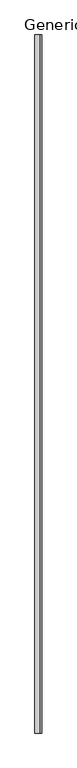
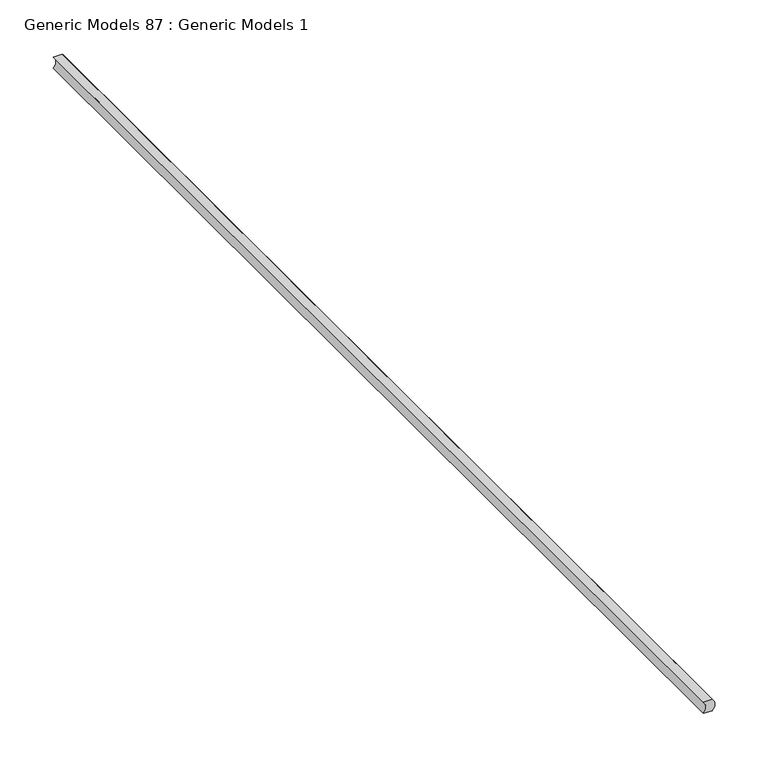
"""IFC4 building model written with IfcOpenShell, lengths in millimetres: proxy geometry, Generic Models 87 : Generic Models 1."""

import ifcopenshell
import ifcopenshell.guid

model = None  # the IFC model being written
_history = None  # IfcOwnerHistory: only IFC2X3 demands one
_inside = {}  # id of a spatial element -> (the spatial element, [elements in it])
_under = {}  # id of a project, library or spatial element -> (it, [spatial elements below it])
_declared = {}  # id of a project -> (the project, [libraries it declares])
_typed = {}  # id of a type object -> (the type object, [elements of that type])
_made_of = {}  # id of a material, layer set ... -> (it, [elements and type objects made of it])


def new_model(schema):
    """Start an empty IFC model of exactly this schema.

    Asked for "IFC4X3", IfcOpenShell would pick the latest addendum, in which some entities
    have other attributes; the version numbers below select the first issue.
    IFC2X3 requires an IfcOwnerHistory on every rooted entity: one is made here for all.
    """
    global model, _history
    if schema == "IFC4X3":
        model = ifcopenshell.file(schema_version=(4, 3, 0, 0))
    else:
        model = ifcopenshell.file(schema=schema)
    _inside.clear()
    _under.clear()
    _declared.clear()
    _typed.clear()
    _made_of.clear()
    _history = None
    if model.schema == "IFC2X3":
        org = make("IfcOrganization", Name="unknown")
        user = make(
            "IfcPersonAndOrganization",
            ThePerson=make("IfcPerson", FamilyName="unknown"),
            TheOrganization=org,
        )
        app = make(
            "IfcApplication",
            ApplicationDeveloper=org,
            Version="unknown",
            ApplicationFullName="unknown",
            ApplicationIdentifier="unknown",
        )
        _history = make(
            "IfcOwnerHistory",
            OwningUser=user,
            OwningApplication=app,
            ChangeAction="ADDED",
            CreationDate=0,
        )
    return model


def make(cls, **values):
    """One entity of the class cls with the attributes given. An attribute that is None is left unset."""
    return model.create_entity(
        cls, **{name: value for name, value in values.items() if value is not None}
    )


def rooted(cls, **values):
    """An entity with a GlobalId (a new one), such as an element, a storey or a relation."""
    return make(cls, GlobalId=ifcopenshell.guid.new(), OwnerHistory=_history, **values)


def si_unit(unit_type, name, prefix=None):
    """IfcSIUnit, for example si_unit("LENGTHUNIT", "METRE", prefix="MILLI")."""
    return make("IfcSIUnit", UnitType=unit_type, Prefix=prefix, Name=name)


def assignment(units):
    """IfcUnitAssignment: the units of a project."""
    return None if units is None else make("IfcUnitAssignment", Units=units)


def point(xyz):
    """IfcCartesianPoint."""
    return None if xyz is None else make("IfcCartesianPoint", Coordinates=xyz)


def direction(xyz):
    """IfcDirection."""
    return None if xyz is None else make("IfcDirection", DirectionRatios=xyz)


def frame(location, z_axis=None, x_axis=None):
    """IfcAxis2Placement3D, a coordinate frame: its origin and axes. An axis left out is left unset."""
    return make(
        "IfcAxis2Placement3D",
        Location=point(location),
        Axis=direction(z_axis),
        RefDirection=direction(x_axis),
    )


def frame_2d(location, x_axis=None):
    """IfcAxis2Placement2D, a coordinate frame in the plane: its origin and x axis."""
    return make(
        "IfcAxis2Placement2D", Location=point(location), RefDirection=direction(x_axis)
    )


def origin():
    """The frame at (0, 0, 0) with its axes left unset."""
    return frame((0.0, 0.0, 0.0))


def place(relative_to, where):
    """IfcLocalPlacement: puts the frame where relative to a parent placement (None: the world)."""
    return make(
        "IfcLocalPlacement", PlacementRelTo=relative_to, RelativePlacement=where
    )


def context(
    kind, dimensions, precision=None, world=None, true_north=None, identifier=None
):
    """IfcGeometricRepresentationContext, for example the 3D "Model" context."""
    return make(
        "IfcGeometricRepresentationContext",
        ContextIdentifier=identifier,
        ContextType=kind,
        CoordinateSpaceDimension=dimensions,
        Precision=precision,
        WorldCoordinateSystem=world,
        TrueNorth=true_north,
    )


def project(units=None, contexts=None):
    """IfcProject with its units and contexts."""
    return rooted(
        "IfcProject",
        Name="project",
        RepresentationContexts=contexts,
        UnitsInContext=assignment(units),
    )


def spatial(cls, under=None, at=None, **own):
    """A site, building, storey or space (cls), placed at a placement, below another one or the project."""
    s = rooted(cls, ObjectPlacement=at, **own)
    if under is not None:
        _under.setdefault(under.id(), (under, []))[1].append(s)
    return s


def polyline(points):
    """IfcPolyline through the points."""
    return make("IfcPolyline", Points=[point(p) for p in points])


def circle_curve(where, radius):
    """IfcCircle in the frame where."""
    return make("IfcCircle", Position=where, Radius=radius)


def trimmed(basis, trim1, trim2, sense, master):
    """IfcTrimmedCurve: the piece of a basis curve between two trims."""
    return make(
        "IfcTrimmedCurve",
        BasisCurve=basis,
        Trim1=trim1,
        Trim2=trim2,
        SenseAgreement=sense,
        MasterRepresentation=master,
    )


def segment(curve, same_sense, transition):
    """IfcCompositeCurveSegment."""
    return make(
        "IfcCompositeCurveSegment",
        Transition=transition,
        SameSense=same_sense,
        ParentCurve=curve,
    )


def composite_curve(segments, self_intersect=None):
    """IfcCompositeCurve: segments joined end to end."""
    return make("IfcCompositeCurve", Segments=segments, SelfIntersect=self_intersect)


def outline(outer, holes=None, kind="AREA"):
    """IfcArbitraryClosedProfileDef: a profile drawn as a closed curve; with holes, ...WithVoids."""
    if holes is None:
        return make("IfcArbitraryClosedProfileDef", ProfileType=kind, OuterCurve=outer)
    return make(
        "IfcArbitraryProfileDefWithVoids",
        ProfileType=kind,
        OuterCurve=outer,
        InnerCurves=holes,
    )


def extrude(swept, where, along, depth):
    """IfcExtrudedAreaSolid: the profile swept, set in the frame where, extruded along a direction by depth."""
    return make(
        "IfcExtrudedAreaSolid",
        SweptArea=swept,
        Position=where,
        ExtrudedDirection=direction(along),
        Depth=depth,
    )


def shape(context_of_items, identifier, shape_type, items):
    """IfcShapeRepresentation: the items that make up one representation, for example the "Body"."""
    return make(
        "IfcShapeRepresentation",
        ContextOfItems=context_of_items,
        RepresentationIdentifier=identifier,
        RepresentationType=shape_type,
        Items=items,
    )


def source(mapping_origin, context_of_items, identifier, shape_type, items):
    """IfcRepresentationMap: a shape defined once, which mapped items show again and again."""
    return make(
        "IfcRepresentationMap",
        MappingOrigin=mapping_origin,
        MappedRepresentation=shape(context_of_items, identifier, shape_type, items),
    )


def transform(
    local_origin,
    x_axis=None,
    y_axis=None,
    z_axis=None,
    scale=None,
    scale2=None,
    scale3=None,
    uniform=True,
):
    """IfcCartesianTransformationOperator3D, or its non-uniform kind. x_axis, y_axis, z_axis: its Axis1, 2, 3."""
    if uniform:
        return make(
            "IfcCartesianTransformationOperator3D",
            Axis1=direction(x_axis),
            Axis2=direction(y_axis),
            LocalOrigin=point(local_origin),
            Scale=scale,
            Axis3=direction(z_axis),
        )
    return make(
        "IfcCartesianTransformationOperator3DnonUniform",
        Axis1=direction(x_axis),
        Axis2=direction(y_axis),
        LocalOrigin=point(local_origin),
        Scale=scale,
        Axis3=direction(z_axis),
        Scale2=scale2,
        Scale3=scale3,
    )


def mapped(mapping_source, mapping_target):
    """IfcMappedItem: shows the shape of a source again, moved by a transform."""
    return make(
        "IfcMappedItem", MappingSource=mapping_source, MappingTarget=mapping_target
    )


def made_of(thing, what):
    """Note that an element or type object is made of a material, layer set ...; save() writes the relation."""
    if what is not None:
        _made_of.setdefault(what.id(), (what, []))[1].append(thing)
    return thing


def element(
    cls,
    number,
    at=None,
    inside=None,
    cuts=None,
    type_object=None,
    material=None,
    context=None,
    identifier="Body",
    shape_type=None,
    held_by="IfcProductDefinitionShape",
    body=None,
    shapes=None,
    **own,
):
    """One element of the class cls, such as IfcWall. Its Tag is "e" and its number.

    at: its placement. inside: the storey or other place that contains it. cuts: it is an
    opening in that element (IfcRelVoidsElement). A single representation is given by context,
    identifier, shape_type and body (its items); several are given by shapes. held_by: the class
    of the entity that holds the representations. save() writes the other relations.
    """
    e = rooted(cls, Tag="e%d" % number, ObjectPlacement=at, **own)
    if body is not None:
        shapes = [shape(context, identifier, shape_type, body)]
    if shapes is not None:
        e.Representation = make(held_by, Representations=shapes)
    if inside is not None:
        _inside.setdefault(inside.id(), (inside, []))[1].append(e)
    if cuts is not None:
        rooted(
            "IfcRelVoidsElement", RelatingBuildingElement=cuts, RelatedOpeningElement=e
        )
    if type_object is not None:
        _typed.setdefault(type_object.id(), (type_object, []))[1].append(e)
    return made_of(e, material)


def aggregate(whole, parts):
    """IfcRelAggregates: a whole, such as a stair, and the parts it consists of."""
    return rooted("IfcRelAggregates", RelatingObject=whole, RelatedObjects=parts)


def save(model, path):
    """Write the relations noted so far, then the file.

    IfcRelAggregates (storeys below a building ...), IfcRelContainedInSpatialStructure (elements
    in a storey), IfcRelDefinesByType, IfcRelAssociatesMaterial and IfcRelDeclares: one each for
    every whole, place, type object, material and project.
    """
    for whole, parts in _under.values():
        aggregate(whole, parts)
    for where, things in _inside.values():
        rooted(
            "IfcRelContainedInSpatialStructure",
            RelatedElements=things,
            RelatingStructure=where,
        )
    for kind, things in _typed.values():
        rooted("IfcRelDefinesByType", RelatedObjects=things, RelatingType=kind)
    for what, things in _made_of.values():
        rooted("IfcRelAssociatesMaterial", RelatedObjects=things, RelatingMaterial=what)
    for by, libraries in _declared.values():
        rooted("IfcRelDeclares", RelatingContext=by, RelatedDefinitions=libraries)
    model.write(path)


def generic_models_87_generic_models_1_0e45ed3c(model_context):
    return source(origin(), model_context, "Body", "SweptSolid", [
        extrude(outline(composite_curve([segment(polyline([(2466.250412, 48444.15), (2466.250412, 48453.675)]), True, "CONTINUOUS"), segment(trimmed(circle_curve(frame_2d((2472.600412, 48447.845519)), 8.620055), [point((2466.250412, 48453.675))], [point((2478.950412, 48453.675))], False, "CARTESIAN"), True, "CONTINUOUS"), segment(polyline([(2478.950412, 48453.675), (2478.950412, 48444.15)]), True, "CONTINUOUS"), segment(trimmed(circle_curve(frame_2d((2472.600412, 48438.320519)), 8.620055), [point((2478.950412, 48444.15))], [point((2466.250412, 48444.15))], True, "CARTESIAN"), True, "CONTINUOUS")], self_intersect=False)), frame((0.0, 0.0, 0.0), z_axis=(0.0, 1.0, 0.0), x_axis=(0.0, 0.0, 1.0)), (0.0, 0.0, 1.0), 1219.2),
    ])


if __name__ == "__main__":
    model = new_model("IFC4")
    model_context = context("Model", 3, world=origin())
    ifc_project = project(units=[si_unit("LENGTHUNIT", "METRE", prefix="MILLI")], contexts=[model_context])
    site = spatial("IfcSite", under=ifc_project)
    building = spatial("IfcBuilding", under=site)
    placement = place(None, origin())
    generic_models_87_generic_models_1_shape = generic_models_87_generic_models_1_0e45ed3c(model_context)
    element("IfcBuildingElementProxy", 1, Name="Generic Models 87 : Generic Models 1", ObjectType="Generic Models 87 : Generic Models 1", at=placement, inside=building, context=model_context, shape_type="MappedRepresentation", body=[
        mapped(generic_models_87_generic_models_1_shape, transform((0.0, 0.0, 0.0), x_axis=(1.0, 0.0, 0.0), y_axis=(0.0, 1.0, 0.0), z_axis=(0.0, 0.0, 1.0))),
    ])
    save(model, "model.ifc")

# Revit data of these elements
# Element 1 (IfcBuildingElementProxy, "Generic Models 87 : Generic Models 1")
#   Materials on its faces: "ACOUSTICAL SEALANT"
# Materials
#   "ACOUSTICAL SEALANT": class "Unassigned", colour RGB 120 120 120, transparency 0, Cost = 0
